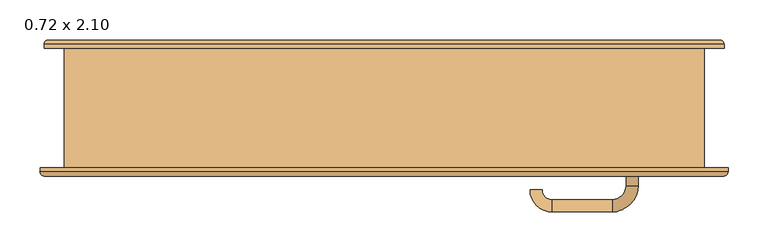
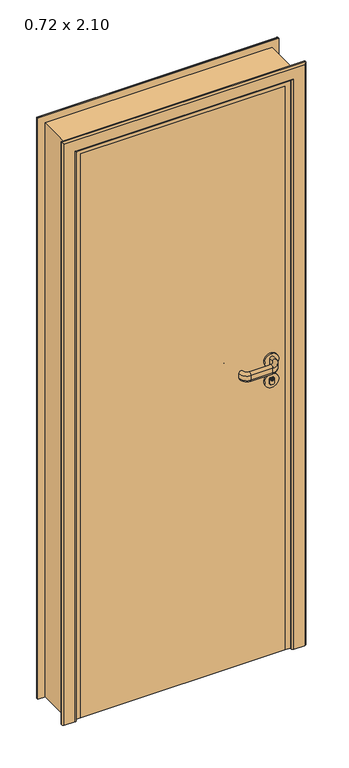
"""IFC4 building model written with IfcOpenShell, lengths in millimetres: door geometry, CC_PORTA ABRIR_1 FOLHA LISA : 0.72 x 2.10."""

import ifcopenshell
import ifcopenshell.guid

model = None  # the IFC model being written
_history = None  # IfcOwnerHistory: only IFC2X3 demands one
_inside = {}  # id of a spatial element -> (the spatial element, [elements in it])
_under = {}  # id of a project, library or spatial element -> (it, [spatial elements below it])
_declared = {}  # id of a project -> (the project, [libraries it declares])
_typed = {}  # id of a type object -> (the type object, [elements of that type])
_made_of = {}  # id of a material, layer set ... -> (it, [elements and type objects made of it])


def new_model(schema):
    """Start an empty IFC model of exactly this schema.

    Asked for "IFC4X3", IfcOpenShell would pick the latest addendum, in which some entities
    have other attributes; the version numbers below select the first issue.
    IFC2X3 requires an IfcOwnerHistory on every rooted entity: one is made here for all.
    """
    global model, _history
    if schema == "IFC4X3":
        model = ifcopenshell.file(schema_version=(4, 3, 0, 0))
    else:
        model = ifcopenshell.file(schema=schema)
    _inside.clear()
    _under.clear()
    _declared.clear()
    _typed.clear()
    _made_of.clear()
    _history = None
    if model.schema == "IFC2X3":
        org = make("IfcOrganization", Name="unknown")
        user = make(
            "IfcPersonAndOrganization",
            ThePerson=make("IfcPerson", FamilyName="unknown"),
            TheOrganization=org,
        )
        app = make(
            "IfcApplication",
            ApplicationDeveloper=org,
            Version="unknown",
            ApplicationFullName="unknown",
            ApplicationIdentifier="unknown",
        )
        _history = make(
            "IfcOwnerHistory",
            OwningUser=user,
            OwningApplication=app,
            ChangeAction="ADDED",
            CreationDate=0,
        )
    return model


def make(cls, **values):
    """One entity of the class cls with the attributes given. An attribute that is None is left unset."""
    return model.create_entity(
        cls, **{name: value for name, value in values.items() if value is not None}
    )


def rooted(cls, **values):
    """An entity with a GlobalId (a new one), such as an element, a storey or a relation."""
    return make(cls, GlobalId=ifcopenshell.guid.new(), OwnerHistory=_history, **values)


def si_unit(unit_type, name, prefix=None):
    """IfcSIUnit, for example si_unit("LENGTHUNIT", "METRE", prefix="MILLI")."""
    return make("IfcSIUnit", UnitType=unit_type, Prefix=prefix, Name=name)


def assignment(units):
    """IfcUnitAssignment: the units of a project."""
    return None if units is None else make("IfcUnitAssignment", Units=units)


def point(xyz):
    """IfcCartesianPoint."""
    return None if xyz is None else make("IfcCartesianPoint", Coordinates=xyz)


def direction(xyz):
    """IfcDirection."""
    return None if xyz is None else make("IfcDirection", DirectionRatios=xyz)


def frame(location, z_axis=None, x_axis=None):
    """IfcAxis2Placement3D, a coordinate frame: its origin and axes. An axis left out is left unset."""
    return make(
        "IfcAxis2Placement3D",
        Location=point(location),
        Axis=direction(z_axis),
        RefDirection=direction(x_axis),
    )


def frame_2d(location, x_axis=None):
    """IfcAxis2Placement2D, a coordinate frame in the plane: its origin and x axis."""
    return make(
        "IfcAxis2Placement2D", Location=point(location), RefDirection=direction(x_axis)
    )


def origin():
    """The frame at (0, 0, 0) with its axes left unset."""
    return frame((0.0, 0.0, 0.0))


def origin_with_axes():
    """The frame at (0, 0, 0) with the z axis (0, 0, 1) and the x axis (1, 0, 0) written out."""
    return frame((0.0, 0.0, 0.0), z_axis=(0.0, 0.0, 1.0), x_axis=(1.0, 0.0, 0.0))


def place(relative_to, where):
    """IfcLocalPlacement: puts the frame where relative to a parent placement (None: the world)."""
    return make(
        "IfcLocalPlacement", PlacementRelTo=relative_to, RelativePlacement=where
    )


def context(
    kind, dimensions, precision=None, world=None, true_north=None, identifier=None
):
    """IfcGeometricRepresentationContext, for example the 3D "Model" context."""
    return make(
        "IfcGeometricRepresentationContext",
        ContextIdentifier=identifier,
        ContextType=kind,
        CoordinateSpaceDimension=dimensions,
        Precision=precision,
        WorldCoordinateSystem=world,
        TrueNorth=true_north,
    )


def project(units=None, contexts=None):
    """IfcProject with its units and contexts."""
    return rooted(
        "IfcProject",
        Name="project",
        RepresentationContexts=contexts,
        UnitsInContext=assignment(units),
    )


def spatial(cls, under=None, at=None, **own):
    """A site, building, storey or space (cls), placed at a placement, below another one or the project."""
    s = rooted(cls, ObjectPlacement=at, **own)
    if under is not None:
        _under.setdefault(under.id(), (under, []))[1].append(s)
    return s


def polyline(points):
    """IfcPolyline through the points."""
    return make("IfcPolyline", Points=[point(p) for p in points])


def circle_curve(where, radius):
    """IfcCircle in the frame where."""
    return make("IfcCircle", Position=where, Radius=radius)


def ellipse_curve(where, semi_axis1, semi_axis2):
    """IfcEllipse in the frame where."""
    return make(
        "IfcEllipse", Position=where, SemiAxis1=semi_axis1, SemiAxis2=semi_axis2
    )


def trimmed(basis, trim1, trim2, sense, master):
    """IfcTrimmedCurve: the piece of a basis curve between two trims."""
    return make(
        "IfcTrimmedCurve",
        BasisCurve=basis,
        Trim1=trim1,
        Trim2=trim2,
        SenseAgreement=sense,
        MasterRepresentation=master,
    )


def segment(curve, same_sense, transition):
    """IfcCompositeCurveSegment."""
    return make(
        "IfcCompositeCurveSegment",
        Transition=transition,
        SameSense=same_sense,
        ParentCurve=curve,
    )


def composite_curve(segments, self_intersect=None):
    """IfcCompositeCurve: segments joined end to end."""
    return make("IfcCompositeCurve", Segments=segments, SelfIntersect=self_intersect)


def outline(outer, holes=None, kind="AREA"):
    """IfcArbitraryClosedProfileDef: a profile drawn as a closed curve; with holes, ...WithVoids."""
    if holes is None:
        return make("IfcArbitraryClosedProfileDef", ProfileType=kind, OuterCurve=outer)
    return make(
        "IfcArbitraryProfileDefWithVoids",
        ProfileType=kind,
        OuterCurve=outer,
        InnerCurves=holes,
    )


def extrude(swept, where, along, depth):
    """IfcExtrudedAreaSolid: the profile swept, set in the frame where, extruded along a direction by depth."""
    return make(
        "IfcExtrudedAreaSolid",
        SweptArea=swept,
        Position=where,
        ExtrudedDirection=direction(along),
        Depth=depth,
    )


def faces_of(points, faces, orient=None, outer=None):
    """IfcFace entities. A face is a list of loops; a loop is a list of indices into points, from 0.

    orient and outer hold one flag for each loop. By default every Orientation is true, the
    first loop of a face is its IfcFaceOuterBound and the others are IfcFaceBound.
    """
    made = []
    for i, loops in enumerate(faces):
        bounds = []
        for j, loop in enumerate(loops):
            is_outer = j == 0 if outer is None else outer[i][j]
            bounds.append(
                make(
                    "IfcFaceOuterBound" if is_outer else "IfcFaceBound",
                    Bound=make("IfcPolyLoop", Polygon=[points[k] for k in loop]),
                    Orientation=True if orient is None else orient[i][j],
                )
            )
        made.append(make("IfcFace", Bounds=bounds))
    return made


def faceted_brep(points, faces, orient=None, outer=None, voids=None):
    """IfcFacetedBrep: a solid bounded by flat faces; with voids (closed shells), ...WithVoids."""
    shared = [point(p) for p in points]
    hull = make("IfcClosedShell", CfsFaces=faces_of(shared, faces, orient, outer))
    if voids is None:
        return make("IfcFacetedBrep", Outer=hull)
    return make(
        "IfcFacetedBrepWithVoids",
        Outer=hull,
        Voids=[
            make(cls, CfsFaces=faces_of(shared, fs, o, b)) for cls, fs, o, b in voids
        ],
    )


def shape(context_of_items, identifier, shape_type, items):
    """IfcShapeRepresentation: the items that make up one representation, for example the "Body"."""
    return make(
        "IfcShapeRepresentation",
        ContextOfItems=context_of_items,
        RepresentationIdentifier=identifier,
        RepresentationType=shape_type,
        Items=items,
    )


def source(mapping_origin, context_of_items, identifier, shape_type, items):
    """IfcRepresentationMap: a shape defined once, which mapped items show again and again."""
    return make(
        "IfcRepresentationMap",
        MappingOrigin=mapping_origin,
        MappedRepresentation=shape(context_of_items, identifier, shape_type, items),
    )


def transform(
    local_origin,
    x_axis=None,
    y_axis=None,
    z_axis=None,
    scale=None,
    scale2=None,
    scale3=None,
    uniform=True,
):
    """IfcCartesianTransformationOperator3D, or its non-uniform kind. x_axis, y_axis, z_axis: its Axis1, 2, 3."""
    if uniform:
        return make(
            "IfcCartesianTransformationOperator3D",
            Axis1=direction(x_axis),
            Axis2=direction(y_axis),
            LocalOrigin=point(local_origin),
            Scale=scale,
            Axis3=direction(z_axis),
        )
    return make(
        "IfcCartesianTransformationOperator3DnonUniform",
        Axis1=direction(x_axis),
        Axis2=direction(y_axis),
        LocalOrigin=point(local_origin),
        Scale=scale,
        Axis3=direction(z_axis),
        Scale2=scale2,
        Scale3=scale3,
    )


def mapped(mapping_source, mapping_target):
    """IfcMappedItem: shows the shape of a source again, moved by a transform."""
    return make(
        "IfcMappedItem", MappingSource=mapping_source, MappingTarget=mapping_target
    )


def made_of(thing, what):
    """Note that an element or type object is made of a material, layer set ...; save() writes the relation."""
    if what is not None:
        _made_of.setdefault(what.id(), (what, []))[1].append(thing)
    return thing


def element(
    cls,
    number,
    at=None,
    inside=None,
    cuts=None,
    type_object=None,
    material=None,
    context=None,
    identifier="Body",
    shape_type=None,
    held_by="IfcProductDefinitionShape",
    body=None,
    shapes=None,
    **own,
):
    """One element of the class cls, such as IfcWall. Its Tag is "e" and its number.

    at: its placement. inside: the storey or other place that contains it. cuts: it is an
    opening in that element (IfcRelVoidsElement). A single representation is given by context,
    identifier, shape_type and body (its items); several are given by shapes. held_by: the class
    of the entity that holds the representations. save() writes the other relations.
    """
    e = rooted(cls, Tag="e%d" % number, ObjectPlacement=at, **own)
    if body is not None:
        shapes = [shape(context, identifier, shape_type, body)]
    if shapes is not None:
        e.Representation = make(held_by, Representations=shapes)
    if inside is not None:
        _inside.setdefault(inside.id(), (inside, []))[1].append(e)
    if cuts is not None:
        rooted(
            "IfcRelVoidsElement", RelatingBuildingElement=cuts, RelatedOpeningElement=e
        )
    if type_object is not None:
        _typed.setdefault(type_object.id(), (type_object, []))[1].append(e)
    return made_of(e, material)


def aggregate(whole, parts):
    """IfcRelAggregates: a whole, such as a stair, and the parts it consists of."""
    return rooted("IfcRelAggregates", RelatingObject=whole, RelatedObjects=parts)


def save(model, path):
    """Write the relations noted so far, then the file.

    IfcRelAggregates (storeys below a building ...), IfcRelContainedInSpatialStructure (elements
    in a storey), IfcRelDefinesByType, IfcRelAssociatesMaterial and IfcRelDeclares: one each for
    every whole, place, type object, material and project.
    """
    for whole, parts in _under.values():
        aggregate(whole, parts)
    for where, things in _inside.values():
        rooted(
            "IfcRelContainedInSpatialStructure",
            RelatedElements=things,
            RelatingStructure=where,
        )
    for kind, things in _typed.values():
        rooted("IfcRelDefinesByType", RelatedObjects=things, RelatingType=kind)
    for what, things in _made_of.values():
        rooted("IfcRelAssociatesMaterial", RelatedObjects=things, RelatingMaterial=what)
    for by, libraries in _declared.values():
        rooted("IfcRelDeclares", RelatingContext=by, RelatedDefinitions=libraries)
    model.write(path)


def plane_surface(at):
    """IfcPlane: the flat surface through the origin of the frame at, square to its z axis."""
    return make("IfcPlane", Position=at)


def cylinder_surface(at, radius):
    """IfcCylindricalSurface: all points at the distance radius from the z axis of the frame at."""
    return make("IfcCylindricalSurface", Position=at, Radius=radius)


def revolved_surface(curve, axis_point, axis_direction):
    """IfcSurfaceOfRevolution: the curve turned about the line through axis_point along axis_direction."""
    return make(
        "IfcSurfaceOfRevolution",
        SweptCurve=make("IfcArbitraryOpenProfileDef", ProfileType="CURVE", Curve=curve),
        AxisPosition=make("IfcAxis1Placement", Location=point(axis_point), Axis=direction(axis_direction)),
    )


def advanced_brep(points, edges, surfaces, faces):
    """IfcAdvancedBrep: a solid bounded by faces that lie on surfaces and meet in shared edges.

    An edge is (start, end): straight between two places in points (the first is 0);
    or (start, end, curve); or (start, end, curve, False) where it runs against its curve.
    A face is (place in surfaces, loops), or (place, loops, False) where it looks against
    its surface's normal. A loop lists edges by number (the first is 1), with a minus sign
    where the edge is run from its end to its start. The first loop is the outer one.
    """
    corners = [point(p) for p in points]
    vertices = [make("IfcVertexPoint", VertexGeometry=c) for c in corners]
    made = []
    for start, end, *more in edges:
        made.append(
            make(
                "IfcEdgeCurve",
                EdgeStart=vertices[start],
                EdgeEnd=vertices[end],
                EdgeGeometry=more[0] if more else make("IfcPolyline", Points=[corners[start], corners[end]]),
                SameSense=more[1] if len(more) > 1 else True,
            )
        )
    hull = []
    for where, loops, *sense in faces:
        bounds = []
        for j, loop in enumerate(loops):
            ring = [make("IfcOrientedEdge", EdgeElement=made[abs(k) - 1], Orientation=k > 0) for k in loop]
            bounds.append(
                make(
                    "IfcFaceOuterBound" if j == 0 else "IfcFaceBound",
                    Bound=make("IfcEdgeLoop", EdgeList=ring),
                    Orientation=True,
                )
            )
        hull.append(make("IfcAdvancedFace", Bounds=bounds, FaceSurface=surfaces[where], SameSense=sense[0] if sense else True))
    return make("IfcAdvancedBrep", Outer=make("IfcClosedShell", CfsFaces=hull))


def door_0_72_x_2_10_8ac540cf(model_context):
    return source(origin(), model_context, "Body", "SolidModel", [
        advanced_brep(
        [(302.5, -40.0, 1091.5062746), (317.5, -40.0, 1091.5062746), (317.5, -40.0, 1108.3826844), (302.5, -40.0, 1108.3826844), (317.5, -18.0, 1091.5062746), (317.5, -18.0, 1108.3826844), (302.5, -18.0, 1108.3826844), (302.5, -18.0, 1091.5062746), (285.0, 14.5, 1108.3826844), (285.0, 14.5, 1091.5062746), (210.0, 14.5, 1091.5062746), (210.0, 14.5, 1108.3826844), (285.0, -0.5, 1091.5062746), (285.0, -0.5, 1108.3826844), (210.0, -0.5, 1108.3826844), (210.0, -0.5, 1091.5062746), (197.5, -13.0, 1091.5062746), (197.5, -13.0, 1108.3826844), (182.5, -13.0, 1108.3826844), (182.5, -13.0, 1091.5062746)],
        [
            (0, 1, circle_curve(frame((310.0, -40.0, 1091.5062746), z_axis=(0.0, -1.0, 0.0), x_axis=(0.0, 0.0, 1.0)), 7.5)),
            (1, 2),
            (2, 3, circle_curve(frame((310.0, -40.0, 1108.3826844), z_axis=(0.0, -1.0, 0.0), x_axis=(0.0, 0.0, 1.0)), 7.5)),
            (3, 0),
            (1, 4),
            (4, 5),
            (5, 2),
            (3, 6),
            (6, 7),
            (7, 0),
            (8, 9),
            (9, 10),
            (10, 11),
            (11, 8),
            (12, 13),
            (13, 14),
            (14, 15),
            (15, 12),
            (7, 4, circle_curve(frame((310.0, -18.0, 1091.5062746), z_axis=(0.0, -1.0, 0.0), x_axis=(0.0, 0.0, 1.0)), 7.5)),
            (5, 6, circle_curve(frame((310.0, -18.0, 1108.3826844), z_axis=(0.0, -1.0, 0.0), x_axis=(0.0, 0.0, 1.0)), 7.5)),
            (9, 12, circle_curve(frame((285.0, 7.0, 1091.5062746), z_axis=(-1.0, 0.0, 0.0), x_axis=(0.0, 0.0, 1.0)), 7.5)),
            (15, 10, circle_curve(frame((210.0, 7.0, 1091.5062746), z_axis=(1.0, 0.0, 0.0), x_axis=(0.0, 0.0, 1.0)), 7.5)),
            (13, 8, circle_curve(frame((285.0, 7.0, 1108.3826844), z_axis=(-1.0, 0.0, 0.0), x_axis=(0.0, 0.0, 1.0)), 7.5)),
            (11, 14, circle_curve(frame((210.0, 7.0, 1108.3826844), z_axis=(1.0, 0.0, 0.0), x_axis=(0.0, 0.0, 1.0)), 7.5)),
            (9, 4, circle_curve(frame((285.0, -18.0, 1091.5062746), z_axis=(0.0, 0.0, -1.0), x_axis=(1.0, 0.0, 0.0)), 32.5)),
            (7, 12, circle_curve(frame((285.0, -18.0, 1091.5062746), z_axis=(0.0, 0.0, 1.0), x_axis=(1.0, 0.0, 0.0)), 17.5)),
            (8, 5, circle_curve(frame((285.0, -18.0, 1108.3826844), z_axis=(0.0, 0.0, -1.0), x_axis=(1.0, 0.0, 0.0)), 32.5)),
            (13, 6, circle_curve(frame((285.0, -18.0, 1108.3826844), z_axis=(0.0, 0.0, -1.0), x_axis=(1.0, 0.0, 0.0)), 17.5)),
            (16, 17),
            (17, 18, circle_curve(frame((190.0, -13.0, 1108.3826844), z_axis=(0.0, -1.0, 0.0), x_axis=(0.0, 0.0, 1.0)), 7.5)),
            (18, 19),
            (19, 16, circle_curve(frame((190.0, -13.0, 1091.5062746), z_axis=(0.0, -1.0, 0.0), x_axis=(0.0, 0.0, 1.0)), 7.5)),
            (19, 10, circle_curve(frame((210.0, -13.0, 1091.5062746), z_axis=(0.0, 0.0, -1.0), x_axis=(0.0, 1.0, 0.0)), 27.5)),
            (15, 16, circle_curve(frame((210.0, -13.0, 1091.5062746), z_axis=(0.0, 0.0, 1.0), x_axis=(0.0, 1.0, 0.0)), 12.5)),
            (18, 11, circle_curve(frame((210.0, -13.0, 1108.3826844), z_axis=(0.0, 0.0, -1.0), x_axis=(0.0, 1.0, 0.0)), 27.5)),
            (17, 14, circle_curve(frame((210.0, -13.0, 1108.3826844), z_axis=(0.0, 0.0, -1.0), x_axis=(0.0, 1.0, 0.0)), 12.5)),
        ],
        [
            plane_surface(frame((310.0, -40.0, 1099.9444795), z_axis=(0.0, -1.0, 0.0), x_axis=(0.0, 0.0, 1.0))),
            plane_surface(frame((317.5, -40.0, 1091.5062746), z_axis=(1.0, 0.0, 0.0), x_axis=(0.0, 1.0, 0.0))),
            plane_surface(frame((302.5, -40.0, 1108.3826844), z_axis=(-1.0, 0.0, 0.0), x_axis=(0.0, 1.0, 0.0))),
            plane_surface(frame((285.0, 14.5, 1091.5062746), z_axis=(0.0, 1.0, 0.0), x_axis=(-1.0, 0.0, 0.0))),
            plane_surface(frame((285.0, -0.5, 1108.3826844), z_axis=(0.0, -1.0, 0.0), x_axis=(-1.0, 0.0, 0.0))),
            cylinder_surface(frame((310.0, -40.0, 1091.5062746), z_axis=(0.0, -1.0, 0.0), x_axis=(0.0, 0.0, 1.0)), 7.5),
            cylinder_surface(frame((310.0, -40.0, 1108.3826844), z_axis=(0.0, -1.0, 0.0), x_axis=(0.0, 0.0, 1.0)), 7.5),
            cylinder_surface(frame((285.0, 7.0, 1091.5062746), z_axis=(1.0, 0.0, 0.0), x_axis=(0.0, 0.0, 1.0)), 7.5),
            cylinder_surface(frame((285.0, 7.0, 1108.3826844), z_axis=(1.0, 0.0, 0.0), x_axis=(0.0, 0.0, 1.0)), 7.5),
            revolved_surface(trimmed(ellipse_curve(frame((310.0, -18.0, 1091.5062746), z_axis=(0.0, -1.0, 0.0), x_axis=(0.0, 0.0, 1.0)), 7.5, 7.5), [point((302.5, -18.0, 1091.5062746))], [point((317.5, -18.0, 1091.5062746))], True, "CARTESIAN"), (285.0, -18.0, 1099.9444795), (0.0, 0.0, 1.0)),
            cylinder_surface(frame((285.0, -18.0, 1099.9444795), z_axis=(0.0, 0.0, 1.0), x_axis=(1.0, 0.0, 0.0)), 32.5),
            revolved_surface(trimmed(ellipse_curve(frame((310.0, -18.0, 1108.3826844), z_axis=(0.0, -1.0, 0.0), x_axis=(0.0, 0.0, 1.0)), 7.5, 7.5), [point((317.5, -18.0, 1108.3826844))], [point((302.5, -18.0, 1108.3826844))], True, "CARTESIAN"), (285.0, -18.0, 1099.9444795), (0.0, 0.0, 1.0)),
            revolved_surface(polyline([(302.5, -18.0, 1108.3826844), (302.5, -18.0, 1091.5062746)]), (285.0, -18.0, 1099.9444795), (0.0, 0.0, 1.0)),
            plane_surface(frame((190.0, -13.0, 1099.9444795), z_axis=(0.0, -1.0, 0.0), x_axis=(0.0, 0.0, 1.0))),
            revolved_surface(trimmed(ellipse_curve(frame((210.0, 7.0, 1091.5062746), z_axis=(1.0, 0.0, 0.0), x_axis=(0.0, 0.0, 1.0)), 7.5, 7.5), [point((210.0, -0.5, 1091.5062746))], [point((210.0, 14.5, 1091.5062746))], True, "CARTESIAN"), (210.0, -13.0, 1099.9444795), (0.0, 0.0, 1.0)),
            cylinder_surface(frame((210.0, -13.0, 1099.9444795), z_axis=(0.0, 0.0, 1.0), x_axis=(0.0, 1.0, 0.0)), 27.5),
            revolved_surface(trimmed(ellipse_curve(frame((210.0, 7.0, 1108.3826844), z_axis=(1.0, 0.0, 0.0), x_axis=(0.0, 0.0, 1.0)), 7.5, 7.5), [point((210.0, 14.5, 1108.3826844))], [point((210.0, -0.5, 1108.3826844))], True, "CARTESIAN"), (210.0, -13.0, 1099.9444795), (0.0, 0.0, 1.0)),
            revolved_surface(polyline([(210.0, -0.5, 1108.3826844), (210.0, -0.5, 1091.5062746)]), (210.0, -13.0, 1099.9444795), (0.0, 0.0, 1.0)),
        ],
        [
            (0, [[1, 2, 3, 4]]),
            (1, [[-2, 5, 6, 7]]),
            (2, [[-4, 8, 9, 10]]),
            (3, [[11, 12, 13, 14]]),
            (4, [[15, 16, 17, 18]]),
            (5, [[-1, -10, 19, -5]]),
            (6, [[-3, -7, 20, -8]]),
            (7, [[21, -18, 22, -12]]),
            (8, [[23, -14, 24, -16]]),
            (9, [[25, -19, 26, -21]]),
            (10, [[27, -6, -25, -11]]),
            (11, [[28, -20, -27, -23]]),
            (12, [[-26, -9, -28, -15]]),
            (13, [[29, 30, 31, 32]]),
            (14, [[33, -22, 34, -32]]),
            (15, [[35, -13, -33, -31]]),
            (16, [[36, -24, -35, -30]]),
            (17, [[-34, -17, -36, -29]]),
        ],
    ),
        extrude(outline(polyline([(311.0, -40.0), (309.0, -40.0), (309.0, -30.9), (311.0, -30.9), (311.0, -40.0)])), frame((0.0, 0.0, 1027.9555433), z_axis=(0.0, 0.0, 1.0), x_axis=(1.0, 0.0, 0.0)), (0.0, 0.0, 1.0), 7.8071257),
        extrude(outline(composite_curve([segment(trimmed(circle_curve(frame_2d((1031.5611613, 310.0)), 5.0), [point((1036.5611613, 310.0))], [point((1026.5611613, 310.0))], False, "CARTESIAN"), True, "CONTINUOUS"), segment(trimmed(circle_curve(frame_2d((1031.5611613, 310.0)), 5.0), [point((1026.5611613, 310.0))], [point((1036.5611613, 310.0))], False, "CARTESIAN"), True, "CONTINUOUS")], self_intersect=False), holes=[polyline([(1035.7626689, 311.0), (1027.9555433, 311.0), (1027.9555433, 309.0), (1035.7626689, 309.0), (1035.7626689, 311.0)])]), frame((0.0, -40.0, 0.0), z_axis=(0.0, 1.0, 0.0), x_axis=(0.0, 0.0, 1.0)), (0.0, 0.0, 1.0), 10.0),
        extrude(outline(composite_curve([segment(polyline([(1033.4817325, 302.5), (1016.4817325, 302.5)]), True, "CONTINUOUS"), segment(trimmed(circle_curve(frame_2d((1016.4817325, 306.5)), 4.0), [point((1016.4817325, 302.5))], [point((1012.4817325, 306.5))], False, "CARTESIAN"), True, "CONTINUOUS"), segment(polyline([(1012.4817325, 306.5), (1012.4817325, 313.5)]), True, "CONTINUOUS"), segment(trimmed(circle_curve(frame_2d((1016.4817325, 313.5)), 4.0), [point((1012.4817325, 313.5))], [point((1016.4817325, 317.5))], False, "CARTESIAN"), True, "CONTINUOUS"), segment(polyline([(1016.4817325, 317.5), (1033.4817325, 317.5)]), True, "CONTINUOUS"), segment(trimmed(circle_curve(frame_2d((1033.4817325, 313.5)), 4.0), [point((1033.4817325, 317.5))], [point((1037.4817325, 313.5))], False, "CARTESIAN"), True, "CONTINUOUS"), segment(polyline([(1037.4817325, 313.5), (1037.4817325, 306.5)]), True, "CONTINUOUS"), segment(trimmed(circle_curve(frame_2d((1033.4817325, 306.5)), 4.0), [point((1037.4817325, 306.5))], [point((1033.4817325, 302.5))], False, "CARTESIAN"), True, "CONTINUOUS")], self_intersect=False)), frame((0.0, -40.0, 0.0), z_axis=(0.0, 1.0, 0.0), x_axis=(0.0, 0.0, 1.0)), (0.0, 0.0, 1.0), 9.0),
        extrude(outline(composite_curve([segment(trimmed(circle_curve(frame_2d((1099.9444795, 310.0)), 25.0), [point((1124.9444795, 310.0))], [point((1074.9444795, 310.0))], False, "CARTESIAN"), True, "CONTINUOUS"), segment(trimmed(circle_curve(frame_2d((1099.9444795, 310.0)), 25.0), [point((1074.9444795, 310.0))], [point((1124.9444795, 310.0))], False, "CARTESIAN"), True, "CONTINUOUS")], self_intersect=False)), frame((0.0, -40.0, 0.0), z_axis=(0.0, 1.0, 0.0), x_axis=(0.0, 0.0, 1.0)), (0.0, 0.0, 1.0), 6.0),
        extrude(outline(composite_curve([segment(trimmed(circle_curve(frame_2d((1024.9444795, 310.0)), 25.0), [point((1049.9444795, 310.0))], [point((999.9444795, 310.0))], False, "CARTESIAN"), True, "CONTINUOUS"), segment(trimmed(circle_curve(frame_2d((1024.9444795, 310.0)), 25.0), [point((999.9444795, 310.0))], [point((1049.9444795, 310.0))], False, "CARTESIAN"), True, "CONTINUOUS")], self_intersect=False), holes=[composite_curve([segment(trimmed(circle_curve(frame_2d((1033.4817325, 313.5)), 4.0), [point((1037.4817325, 313.5))], [point((1033.4817325, 317.5))], True, "CARTESIAN"), True, "CONTINUOUS"), segment(polyline([(1033.4817325, 317.5), (1016.4817325, 317.5)]), True, "CONTINUOUS"), segment(trimmed(circle_curve(frame_2d((1016.4817325, 313.5)), 4.0), [point((1016.4817325, 317.5))], [point((1012.4817325, 313.5))], True, "CARTESIAN"), True, "CONTINUOUS"), segment(polyline([(1012.4817325, 313.5), (1012.4817325, 306.5)]), True, "CONTINUOUS"), segment(trimmed(circle_curve(frame_2d((1016.4817325, 306.5)), 4.0), [point((1012.4817325, 306.5))], [point((1016.4817325, 302.5))], True, "CARTESIAN"), True, "CONTINUOUS"), segment(polyline([(1016.4817325, 302.5), (1033.4817325, 302.5)]), True, "CONTINUOUS"), segment(trimmed(circle_curve(frame_2d((1033.4817325, 306.5)), 4.0), [point((1033.4817325, 302.5))], [point((1037.4817325, 306.5))], True, "CARTESIAN"), True, "CONTINUOUS"), segment(polyline([(1037.4817325, 306.5), (1037.4817325, 313.5)]), True, "CONTINUOUS")], self_intersect=False)]), frame((0.0, -40.0, 0.0), z_axis=(0.0, 1.0, 0.0), x_axis=(0.0, 0.0, 1.0)), (0.0, 0.0, 1.0), 6.0),
        extrude(outline(polyline([(311.0, -84.1), (309.0, -84.1), (309.0, -75.0), (311.0, -75.0), (311.0, -84.1)])), frame((0.0, 0.0, 1027.9555433), z_axis=(0.0, 0.0, 1.0), x_axis=(1.0, 0.0, 0.0)), (0.0, 0.0, 1.0), 7.8071257),
        advanced_brep(
        [(310.0, -85.0, 1036.5611613), (310.0, -85.0, 1026.5611613), (311.0, -85.0, 1035.7626689), (311.0, -85.0, 1027.9555433), (309.0, -85.0, 1027.9555433), (309.0, -85.0, 1035.7626689), (310.0, -75.0, 1049.9444795), (310.0, -75.0, 999.9444795), (310.0, -84.0, 1036.5611613), (310.0, -84.0, 1026.5611613), (311.0, -84.0, 1035.7626689), (311.0, -84.0, 1027.9555433), (309.0, -84.0, 1027.9555433), (309.0, -84.0, 1035.7626689), (302.5, -84.0, 1033.4817325), (302.5, -84.0, 1016.4817325), (306.5, -84.0, 1012.4817325), (313.5, -84.0, 1012.4817325), (317.5, -84.0, 1016.4817325), (317.5, -84.0, 1033.4817325), (313.5, -84.0, 1037.4817325), (306.5, -84.0, 1037.4817325), (302.5, -81.0, 1033.4817325), (302.5, -81.0, 1016.4817325), (306.5, -81.0, 1012.4817325), (313.5, -81.0, 1012.4817325), (317.5, -81.0, 1016.4817325), (317.5, -81.0, 1033.4817325), (313.5, -81.0, 1037.4817325), (306.5, -81.0, 1037.4817325), (310.0, -81.0, 1049.9444795), (310.0, -81.0, 999.9444795)],
        [
            (0, 1, circle_curve(frame((310.0, -85.0, 1031.5611613), z_axis=(0.0, -1.0, 0.0), x_axis=(0.0, 0.0, -1.0)), 5.0)),
            (1, 0, circle_curve(frame((310.0, -85.0, 1031.5611613), z_axis=(0.0, -1.0, 0.0), x_axis=(0.0, 0.0, -1.0)), 5.0)),
            (2, 3),
            (3, 4),
            (4, 5),
            (5, 2),
            (6, 7, circle_curve(frame((310.0, -75.0, 1024.9444795), z_axis=(0.0, 1.0, 0.0), x_axis=(0.0, 0.0, -1.0)), 25.0)),
            (7, 6, circle_curve(frame((310.0, -75.0, 1024.9444795), z_axis=(0.0, 1.0, 0.0), x_axis=(0.0, 0.0, -1.0)), 25.0)),
            (0, 8),
            (8, 9, circle_curve(frame((310.0, -84.0, 1031.5611613), z_axis=(0.0, -1.0, 0.0), x_axis=(0.0, 0.0, -1.0)), 5.0)),
            (9, 1),
            (9, 8, circle_curve(frame((310.0, -84.0, 1031.5611613), z_axis=(0.0, -1.0, 0.0), x_axis=(0.0, 0.0, -1.0)), 5.0)),
            (2, 10),
            (10, 11),
            (11, 3),
            (11, 12),
            (12, 4),
            (12, 13),
            (13, 5),
            (13, 10),
            (14, 15),
            (15, 16, circle_curve(frame((306.5, -84.0, 1016.4817325), z_axis=(0.0, -1.0, 0.0), x_axis=(0.0, 0.0, -1.0)), 4.0)),
            (16, 17),
            (17, 18, circle_curve(frame((313.5, -84.0, 1016.4817325), z_axis=(0.0, -1.0, 0.0), x_axis=(0.0, 0.0, -1.0)), 4.0)),
            (18, 19),
            (19, 20, circle_curve(frame((313.5, -84.0, 1033.4817325), z_axis=(0.0, -1.0, 0.0), x_axis=(0.0, 0.0, -1.0)), 4.0)),
            (20, 21),
            (21, 14, circle_curve(frame((306.5, -84.0, 1033.4817325), z_axis=(0.0, -1.0, 0.0), x_axis=(0.0, 0.0, -1.0)), 4.0)),
            (14, 22),
            (22, 23),
            (23, 15),
            (23, 24, circle_curve(frame((306.5, -81.0, 1016.4817325), z_axis=(0.0, -1.0, 0.0), x_axis=(0.0, 0.0, -1.0)), 4.0)),
            (24, 16),
            (24, 25),
            (25, 17),
            (25, 26, circle_curve(frame((313.5, -81.0, 1016.4817325), z_axis=(0.0, -1.0, 0.0), x_axis=(0.0, 0.0, -1.0)), 4.0)),
            (26, 18),
            (26, 27),
            (27, 19),
            (27, 28, circle_curve(frame((313.5, -81.0, 1033.4817325), z_axis=(0.0, -1.0, 0.0), x_axis=(0.0, 0.0, -1.0)), 4.0)),
            (28, 20),
            (28, 29),
            (29, 21),
            (29, 22, circle_curve(frame((306.5, -81.0, 1033.4817325), z_axis=(0.0, -1.0, 0.0), x_axis=(0.0, 0.0, -1.0)), 4.0)),
            (30, 31, circle_curve(frame((310.0, -81.0, 1024.9444795), z_axis=(0.0, -1.0, 0.0), x_axis=(0.0, 0.0, -1.0)), 25.0)),
            (31, 30, circle_curve(frame((310.0, -81.0, 1024.9444795), z_axis=(0.0, -1.0, 0.0), x_axis=(0.0, 0.0, -1.0)), 25.0)),
            (30, 6),
            (7, 31),
        ],
        [
            plane_surface(frame((310.0, -85.0, 1026.5611613), z_axis=(0.0, -1.0, 0.0), x_axis=(1.0, 0.0, 0.0))),
            plane_surface(frame((310.0, -75.0, 1026.5611613), z_axis=(0.0, 1.0, 0.0), x_axis=(-1.0, 0.0, 0.0))),
            cylinder_surface(frame((310.0, -75.0, 1031.5611613), z_axis=(0.0, -1.0, 0.0), x_axis=(0.0, 0.0, -1.0)), 5.0),
            plane_surface(frame((311.0, -85.0, 1035.7626689), z_axis=(-1.0, 0.0, 0.0), x_axis=(0.0, 1.0, 0.0))),
            plane_surface(frame((311.0, -85.0, 1027.9555433), z_axis=(0.0, 0.0, 1.0), x_axis=(0.0, 1.0, 0.0))),
            plane_surface(frame((309.0, -85.0, 1027.9555433), z_axis=(1.0, 0.0, 0.0), x_axis=(0.0, 1.0, 0.0))),
            plane_surface(frame((309.0, -85.0, 1035.7626689), z_axis=(0.0, 0.0, -1.0), x_axis=(0.0, 1.0, 0.0))),
            plane_surface(frame((302.5, -84.0, 1016.4817325), z_axis=(0.0, -1.0, 0.0), x_axis=(0.0, 0.0, -1.0))),
            plane_surface(frame((302.5, -84.0, 1033.4817325), z_axis=(-1.0, 0.0, 0.0), x_axis=(0.0, 1.0, 0.0))),
            cylinder_surface(frame((306.5, -75.0, 1016.4817325), z_axis=(0.0, -1.0, 0.0), x_axis=(0.0, 0.0, -1.0)), 4.0),
            plane_surface(frame((306.5, -84.0, 1012.4817325), z_axis=(0.0, 0.0, -1.0), x_axis=(0.0, 1.0, 0.0))),
            cylinder_surface(frame((313.5, -75.0, 1016.4817325), z_axis=(0.0, -1.0, 0.0), x_axis=(0.0, 0.0, -1.0)), 4.0),
            plane_surface(frame((317.5, -84.0, 1016.4817325), z_axis=(1.0, 0.0, 0.0), x_axis=(0.0, 1.0, 0.0))),
            cylinder_surface(frame((313.5, -75.0, 1033.4817325), z_axis=(0.0, -1.0, 0.0), x_axis=(0.0, 0.0, -1.0)), 4.0),
            plane_surface(frame((313.5, -84.0, 1037.4817325), z_axis=(0.0, 0.0, 1.0), x_axis=(0.0, 1.0, 0.0))),
            cylinder_surface(frame((306.5, -75.0, 1033.4817325), z_axis=(0.0, -1.0, 0.0), x_axis=(0.0, 0.0, -1.0)), 4.0),
            plane_surface(frame((310.0, -81.0, 1074.9444795), z_axis=(0.0, -1.0, 0.0), x_axis=(1.0, 0.0, 0.0))),
            cylinder_surface(frame((310.0, -75.0, 1024.9444795), z_axis=(0.0, -1.0, 0.0), x_axis=(0.0, 0.0, -1.0)), 25.0),
        ],
        [
            (0, [[1, 2], [3, 4, 5, 6]]),
            (1, [[7, 8]]),
            (2, [[-1, 9, 10, 11]]),
            (2, [[-2, -11, 12, -9]]),
            (3, [[-3, 13, 14, 15]]),
            (4, [[-4, -15, 16, 17]]),
            (5, [[-5, -17, 18, 19]]),
            (6, [[-6, -19, 20, -13]]),
            (7, [[-14, -20, -18, -16]]),
            (7, [[21, 22, 23, 24, 25, 26, 27, 28], [-10, -12]]),
            (8, [[-21, 29, 30, 31]]),
            (9, [[-22, -31, 32, 33]]),
            (10, [[-23, -33, 34, 35]]),
            (11, [[-24, -35, 36, 37]]),
            (12, [[-25, -37, 38, 39]]),
            (13, [[-26, -39, 40, 41]]),
            (14, [[-27, -41, 42, 43]]),
            (15, [[-28, -43, 44, -29]]),
            (16, [[45, 46], [-30, -44, -42, -40, -38, -36, -34, -32]]),
            (17, [[-45, 47, -8, 48]]),
            (17, [[-46, -48, -7, -47]]),
        ],
    ),
        advanced_brep(
        [(310.0, -75.0, 1124.9444795), (310.0, -75.0, 1074.9444795), (310.0, -81.0, 1124.9444795), (310.0, -81.0, 1074.9444795)],
        [
            (0, 1, circle_curve(frame((310.0, -75.0, 1099.9444795), z_axis=(0.0, 1.0, 0.0), x_axis=(0.0, 0.0, -1.0)), 25.0)),
            (1, 0, circle_curve(frame((310.0, -75.0, 1099.9444795), z_axis=(0.0, 1.0, 0.0), x_axis=(0.0, 0.0, -1.0)), 25.0)),
            (2, 3, circle_curve(frame((310.0, -81.0, 1099.9444795), z_axis=(0.0, -1.0, 0.0), x_axis=(0.0, 0.0, -1.0)), 25.0)),
            (3, 2, circle_curve(frame((310.0, -81.0, 1099.9444795), z_axis=(0.0, -1.0, 0.0), x_axis=(0.0, 0.0, -1.0)), 25.0)),
            (2, 0),
            (1, 3),
        ],
        [
            plane_surface(frame((310.0, -75.0, 1026.5611613), z_axis=(0.0, 1.0, 0.0), x_axis=(-1.0, 0.0, 0.0))),
            plane_surface(frame((310.0, -81.0, 1074.9444795), z_axis=(0.0, -1.0, 0.0), x_axis=(1.0, 0.0, 0.0))),
            cylinder_surface(frame((310.0, -75.0, 1099.9444795), z_axis=(0.0, -1.0, 0.0), x_axis=(0.0, 0.0, -1.0)), 25.0),
        ],
        [
            (0, [[1, 2]]),
            (1, [[3, 4]]),
            (2, [[-3, 5, -2, 6]]),
            (2, [[-4, -6, -1, -5]]),
        ],
    ),
        advanced_brep(
        [(302.5, -75.0, 1108.4382049), (317.5, -75.0, 1108.4382049), (317.5, -75.0, 1091.5617951), (302.5, -75.0, 1091.5617951), (317.5, -97.0, 1108.4382049), (317.5, -97.0, 1091.5617951), (302.5, -97.0, 1091.5617951), (302.5, -97.0, 1108.4382049), (285.0, -129.5, 1091.5617951), (285.0, -129.5, 1108.4382049), (210.0, -129.5, 1108.4382049), (210.0, -129.5, 1091.5617951), (285.0, -114.5, 1108.4382049), (285.0, -114.5, 1091.5617951), (210.0, -114.5, 1091.5617951), (210.0, -114.5, 1108.4382049), (197.5, -102.0, 1108.4382049), (197.5, -102.0, 1091.5617951), (182.5, -102.0, 1091.5617951), (182.5, -102.0, 1108.4382049)],
        [
            (0, 1, circle_curve(frame((310.0, -75.0, 1108.4382049), z_axis=(0.0, 1.0, 0.0), x_axis=(-1.0, 0.0, 0.0)), 7.5)),
            (1, 2),
            (2, 3, circle_curve(frame((310.0, -75.0, 1091.5617951), z_axis=(0.0, 1.0, 0.0), x_axis=(-1.0, 0.0, 0.0)), 7.5)),
            (3, 0),
            (1, 4),
            (4, 5),
            (5, 2),
            (3, 6),
            (6, 7),
            (7, 0),
            (8, 9),
            (9, 10),
            (10, 11),
            (11, 8),
            (12, 13),
            (13, 14),
            (14, 15),
            (15, 12),
            (7, 4, circle_curve(frame((310.0, -97.0, 1108.4382049), z_axis=(0.0, 1.0, 0.0), x_axis=(-1.0, 0.0, 0.0)), 7.5)),
            (5, 6, circle_curve(frame((310.0, -97.0, 1091.5617951), z_axis=(0.0, 1.0, 0.0), x_axis=(-1.0, 0.0, 0.0)), 7.5)),
            (9, 12, circle_curve(frame((285.0, -122.0, 1108.4382049), z_axis=(-1.0, 0.0, 0.0), x_axis=(0.0, 1.0, 0.0)), 7.5)),
            (15, 10, circle_curve(frame((210.0, -122.0, 1108.4382049), z_axis=(1.0, 0.0, 0.0), x_axis=(0.0, 1.0, 0.0)), 7.5)),
            (13, 8, circle_curve(frame((285.0, -122.0, 1091.5617951), z_axis=(-1.0, 0.0, 0.0), x_axis=(0.0, 1.0, 0.0)), 7.5)),
            (11, 14, circle_curve(frame((210.0, -122.0, 1091.5617951), z_axis=(1.0, 0.0, 0.0), x_axis=(0.0, 1.0, 0.0)), 7.5)),
            (9, 4, circle_curve(frame((285.0, -97.0, 1108.4382049), z_axis=(0.0, 0.0, 1.0), x_axis=(1.0, 0.0, 0.0)), 32.5)),
            (7, 12, circle_curve(frame((285.0, -97.0, 1108.4382049), z_axis=(0.0, 0.0, -1.0), x_axis=(1.0, 0.0, 0.0)), 17.5)),
            (8, 5, circle_curve(frame((285.0, -97.0, 1091.5617951), z_axis=(0.0, 0.0, 1.0), x_axis=(1.0, 0.0, 0.0)), 32.5)),
            (13, 6, circle_curve(frame((285.0, -97.0, 1091.5617951), z_axis=(0.0, 0.0, 1.0), x_axis=(1.0, 0.0, 0.0)), 17.5)),
            (16, 17),
            (17, 18, circle_curve(frame((190.0, -102.0, 1091.5617951), z_axis=(0.0, 1.0, 0.0), x_axis=(1.0, 0.0, 0.0)), 7.5)),
            (18, 19),
            (19, 16, circle_curve(frame((190.0, -102.0, 1108.4382049), z_axis=(0.0, 1.0, 0.0), x_axis=(1.0, 0.0, 0.0)), 7.5)),
            (19, 10, circle_curve(frame((210.0, -102.0, 1108.4382049), z_axis=(0.0, 0.0, 1.0), x_axis=(0.0, -1.0, 0.0)), 27.5)),
            (15, 16, circle_curve(frame((210.0, -102.0, 1108.4382049), z_axis=(0.0, 0.0, -1.0), x_axis=(0.0, -1.0, 0.0)), 12.5)),
            (18, 11, circle_curve(frame((210.0, -102.0, 1091.5617951), z_axis=(0.0, 0.0, 1.0), x_axis=(0.0, -1.0, 0.0)), 27.5)),
            (17, 14, circle_curve(frame((210.0, -102.0, 1091.5617951), z_axis=(0.0, 0.0, 1.0), x_axis=(0.0, -1.0, 0.0)), 12.5)),
        ],
        [
            plane_surface(frame((310.0, -75.0, 1100.0), z_axis=(0.0, 1.0, 0.0), x_axis=(0.0, 0.0, -1.0))),
            plane_surface(frame((317.5, -75.0, 1108.4382049), z_axis=(1.0, 0.0, 0.0), x_axis=(0.0, -1.0, 0.0))),
            plane_surface(frame((302.5, -75.0, 1091.5617951), z_axis=(-1.0, 0.0, 0.0), x_axis=(0.0, -1.0, 0.0))),
            plane_surface(frame((285.0, -129.5, 1108.4382049), z_axis=(0.0, -1.0, 0.0), x_axis=(-1.0, 0.0, 0.0))),
            plane_surface(frame((285.0, -114.5, 1091.5617951), z_axis=(0.0, 1.0, 0.0), x_axis=(-1.0, 0.0, 0.0))),
            cylinder_surface(frame((310.0, -75.0, 1108.4382049), z_axis=(0.0, 1.0, 0.0), x_axis=(-1.0, 0.0, 0.0)), 7.5),
            cylinder_surface(frame((310.0, -75.0, 1091.5617951), z_axis=(0.0, 1.0, 0.0), x_axis=(-1.0, 0.0, 0.0)), 7.5),
            cylinder_surface(frame((285.0, -122.0, 1108.4382049), z_axis=(1.0, 0.0, 0.0), x_axis=(0.0, 1.0, 0.0)), 7.5),
            cylinder_surface(frame((285.0, -122.0, 1091.5617951), z_axis=(1.0, 0.0, 0.0), x_axis=(0.0, 1.0, 0.0)), 7.5),
            revolved_surface(trimmed(ellipse_curve(frame((310.0, -97.0, 1108.4382049), z_axis=(0.0, 1.0, 0.0), x_axis=(-1.0, 0.0, 0.0)), 7.5, 7.5), [point((302.5, -97.0, 1108.4382049))], [point((317.5, -97.0, 1108.4382049))], True, "CARTESIAN"), (285.0, -97.0, 1100.0), (0.0, 0.0, -1.0)),
            cylinder_surface(frame((285.0, -97.0, 1100.0), z_axis=(0.0, 0.0, -1.0), x_axis=(1.0, 0.0, 0.0)), 32.5),
            revolved_surface(trimmed(ellipse_curve(frame((310.0, -97.0, 1091.5617951), z_axis=(0.0, 1.0, 0.0), x_axis=(-1.0, 0.0, 0.0)), 7.5, 7.5), [point((317.5, -97.0, 1091.5617951))], [point((302.5, -97.0, 1091.5617951))], True, "CARTESIAN"), (285.0, -97.0, 1100.0), (0.0, 0.0, -1.0)),
            revolved_surface(polyline([(302.5, -97.0, 1091.5617951), (302.5, -97.0, 1108.4382049)]), (285.0, -97.0, 1100.0), (0.0, 0.0, -1.0)),
            plane_surface(frame((190.0, -102.0, 1100.0), z_axis=(0.0, 1.0, 0.0), x_axis=(0.0, 0.0, -1.0))),
            revolved_surface(trimmed(ellipse_curve(frame((210.0, -122.0, 1108.4382049), z_axis=(1.0, 0.0, 0.0), x_axis=(0.0, 1.0, 0.0)), 7.5, 7.5), [point((210.0, -114.5, 1108.4382049))], [point((210.0, -129.5, 1108.4382049))], True, "CARTESIAN"), (210.0, -102.0, 1100.0), (0.0, 0.0, -1.0)),
            cylinder_surface(frame((210.0, -102.0, 1100.0), z_axis=(0.0, 0.0, -1.0), x_axis=(0.0, -1.0, 0.0)), 27.5),
            revolved_surface(trimmed(ellipse_curve(frame((210.0, -122.0, 1091.5617951), z_axis=(1.0, 0.0, 0.0), x_axis=(0.0, 1.0, 0.0)), 7.5, 7.5), [point((210.0, -129.5, 1091.5617951))], [point((210.0, -114.5, 1091.5617951))], True, "CARTESIAN"), (210.0, -102.0, 1100.0), (0.0, 0.0, -1.0)),
            revolved_surface(polyline([(210.0, -114.5, 1091.5617951), (210.0, -114.5, 1108.4382049)]), (210.0, -102.0, 1100.0), (0.0, 0.0, -1.0)),
        ],
        [
            (0, [[1, 2, 3, 4]]),
            (1, [[-2, 5, 6, 7]]),
            (2, [[-4, 8, 9, 10]]),
            (3, [[11, 12, 13, 14]]),
            (4, [[15, 16, 17, 18]]),
            (5, [[-1, -10, 19, -5]]),
            (6, [[-3, -7, 20, -8]]),
            (7, [[21, -18, 22, -12]]),
            (8, [[23, -14, 24, -16]]),
            (9, [[25, -19, 26, -21]]),
            (10, [[27, -6, -25, -11]]),
            (11, [[28, -20, -27, -23]]),
            (12, [[-26, -9, -28, -15]]),
            (13, [[29, 30, 31, 32]]),
            (14, [[33, -22, 34, -32]]),
            (15, [[35, -13, -33, -31]]),
            (16, [[36, -24, -35, -30]]),
            (17, [[-34, -17, -36, -29]]),
        ],
    ),
        extrude(outline(polyline([(360.0, -75.0), (-360.0, -75.0), (-360.0, -40.0), (360.0, -40.0), (360.0, -75.0)])), origin_with_axes(), (0.0, 0.0, 1.0), 2100.0),
        advanced_brep(
        [(-380.5, 85.0, 0.0), (-375.0, 79.5, 0.0), (-375.0, 75.0, 0.0), (-425.0, 75.0, 0.0), (-425.0, 79.500573, 0.0), (-419.500573, 85.0, 0.0), (-380.5, 85.0, 2120.5), (-375.0, 79.5, 2115.0), (-375.0, 75.0, 2115.0), (375.0, 75.0, 2115.0), (375.0, 75.0, 0.0), (425.0, 75.0, 0.0), (425.0, 75.0, 2165.0), (-425.0, 75.0, 2165.0), (-425.0, 79.500573, 2165.0), (-419.500573, 85.0, 2159.500573), (419.500573, 85.0, 2159.500573), (419.500573, 85.0, 0.0), (380.5, 85.0, 0.0), (380.5, 85.0, 2120.5), (375.0, 79.5, 2115.0), (375.0, 79.5, 0.0), (425.0, 79.500573, 0.0), (425.0, 79.500573, 2165.0)],
        [
            (0, 1, circle_curve(frame((-380.5, 79.5, 0.0), z_axis=(0.0, 0.0, -1.0), x_axis=(0.0, 1.0, 0.0)), 5.5)),
            (1, 2),
            (2, 3),
            (3, 4),
            (4, 5, circle_curve(frame((-419.500573, 79.500573, 0.0), z_axis=(0.0, 0.0, -1.0), x_axis=(0.0, 1.0, 0.0)), 5.499427)),
            (5, 0),
            (0, 6),
            (6, 7, ellipse_curve(frame((-380.5, 79.5, 2120.5), z_axis=(-0.7071067811865475, 0.0, -0.7071067811865476), x_axis=(0.7071067811865476, 0.0, -0.7071067811865474)), 7.7781746, 5.5)),
            (7, 1),
            (7, 8),
            (8, 2),
            (8, 9),
            (9, 10),
            (10, 11),
            (11, 12),
            (12, 13),
            (13, 3),
            (13, 14),
            (14, 4),
            (14, 15, ellipse_curve(frame((-419.500573, 79.500573, 2159.500573), z_axis=(-0.7071067811865475, 0.0, -0.7071067811865476), x_axis=(0.7071067811865476, 0.0, -0.7071067811865474)), 7.7773642, 5.499427)),
            (15, 5),
            (15, 16),
            (16, 17),
            (17, 18),
            (18, 19),
            (19, 6),
            (9, 20),
            (20, 21),
            (21, 10),
            (17, 22, circle_curve(frame((419.500573, 79.500573, 0.0), z_axis=(0.0, 0.0, -1.0), x_axis=(0.0, 1.0, 0.0)), 5.499427)),
            (22, 11),
            (21, 18, circle_curve(frame((380.5, 79.5, 0.0), z_axis=(0.0, 0.0, -1.0), x_axis=(0.0, 1.0, 0.0)), 5.5)),
            (23, 12),
            (22, 23),
            (16, 23, ellipse_curve(frame((419.500573, 79.500573, 2159.500573), z_axis=(0.7071067811865475, 0.0, -0.7071067811865475), x_axis=(0.7071067811865474, 0.0, 0.7071067811865477)), 7.7773642, 5.499427)),
            (20, 19, ellipse_curve(frame((380.5, 79.5, 2120.5), z_axis=(0.7071067811865475, 0.0, -0.7071067811865475), x_axis=(0.7071067811865474, 0.0, 0.7071067811865477)), 7.7781746, 5.5)),
            (20, 7),
            (23, 14),
        ],
        [
            plane_surface(frame((-400.0, 75.0, 0.0), z_axis=(0.0, 0.0, -1.0), x_axis=(-1.0, 0.0, 0.0))),
            cylinder_surface(frame((-380.5, 79.5, 0.0), z_axis=(0.0, 0.0, -1.0), x_axis=(0.0, 1.0, 0.0)), 5.5),
            plane_surface(frame((-375.0, 79.5, 0.0), z_axis=(1.0, 0.0, 0.0), x_axis=(0.0, 0.0, 1.0))),
            plane_surface(frame((-375.0, 75.0, 0.0), z_axis=(0.0, -1.0, 0.0), x_axis=(0.0, 0.0, 1.0))),
            plane_surface(frame((-425.0, 75.0, 0.0), z_axis=(-1.0, 0.0, 0.0), x_axis=(0.0, 0.0, 1.0))),
            cylinder_surface(frame((-419.500573, 79.500573, 0.0), z_axis=(0.0, 0.0, -1.0), x_axis=(0.0, 1.0, 0.0)), 5.499427),
            plane_surface(frame((-419.500573, 85.0, 0.0), z_axis=(0.0, 1.0, 0.0), x_axis=(0.0, 0.0, 1.0))),
            plane_surface(frame((375.0, 79.5, 2115.0), z_axis=(-1.0, 0.0, 0.0), x_axis=(0.0, 0.0, -1.0))),
            plane_surface(frame((400.0, 75.0, 0.0), z_axis=(0.0, 0.0, -1.0), x_axis=(1.0, 0.0, 0.0))),
            plane_surface(frame((425.0, 75.0, 2165.0), z_axis=(1.0, 0.0, 0.0), x_axis=(0.0, 0.0, -1.0))),
            cylinder_surface(frame((419.500573, 79.500573, 2140.0), z_axis=(0.0, 0.0, 1.0), x_axis=(0.0, 1.0, 0.0)), 5.499427),
            cylinder_surface(frame((380.5, 79.5, 2140.0), z_axis=(0.0, 0.0, 1.0), x_axis=(0.0, 1.0, 0.0)), 5.5),
            cylinder_surface(frame((-400.0, 79.5, 2120.5), z_axis=(-1.0, 0.0, 0.0), x_axis=(0.0, 1.0, 0.0)), 5.5),
            plane_surface(frame((-375.0, 79.5, 2115.0), z_axis=(0.0, 0.0, -1.0), x_axis=(1.0, 0.0, 0.0))),
            plane_surface(frame((-425.0, 75.0, 2165.0), z_axis=(0.0, 0.0, 1.0), x_axis=(1.0, 0.0, 0.0))),
            cylinder_surface(frame((-400.0, 79.500573, 2159.500573), z_axis=(-1.0, 0.0, 0.0), x_axis=(0.0, 1.0, 0.0)), 5.499427),
        ],
        [
            (0, [[1, 2, 3, 4, 5, 6]]),
            (1, [[-1, 7, 8, 9]]),
            (2, [[-2, -9, 10, 11]]),
            (3, [[-3, -11, 12, 13, 14, 15, 16, 17]]),
            (4, [[-4, -17, 18, 19]]),
            (5, [[-5, -19, 20, 21]]),
            (6, [[-6, -21, 22, 23, 24, 25, 26, -7]]),
            (7, [[27, 28, 29, -13]]),
            (8, [[-24, 30, 31, -14, -29, 32]]),
            (9, [[33, -15, -31, 34]]),
            (10, [[35, -34, -30, -23]]),
            (11, [[36, -25, -32, -28]]),
            (12, [[-8, -26, -36, 37]]),
            (13, [[-10, -37, -27, -12]]),
            (14, [[-18, -16, -33, 38]]),
            (15, [[-20, -38, -35, -22]]),
        ],
    ),
        advanced_brep(
        [(-380.0, -75.0, 0.0), (-380.0, -79.5, 0.0), (-385.5, -85.0, 0.0), (-424.5, -85.0, 0.0), (-430.0, -79.5, 0.0), (-430.0, -75.0, 0.0), (-380.0, -75.0, 2120.0), (-380.0, -79.5, 2120.0), (-385.5, -85.0, 2125.5), (385.5, -85.0, 2125.5), (385.5, -85.0, 0.0), (424.5, -85.0, 0.0), (424.5, -85.0, 2164.5), (-424.5, -85.0, 2164.5), (-430.0, -79.5, 2170.0), (-430.0, -75.0, 2170.0), (430.0, -75.0, 2170.0), (430.0, -75.0, 0.0), (380.0, -75.0, 0.0), (380.0, -75.0, 2120.0), (380.0, -79.5, 2120.0), (380.0, -79.5, 0.0), (430.0, -79.5, 0.0), (430.0, -79.5, 2170.0)],
        [
            (0, 1),
            (1, 2, circle_curve(frame((-385.5, -79.5, 0.0), z_axis=(0.0, 0.0, -1.0), x_axis=(0.0, 1.0, 0.0)), 5.5)),
            (2, 3),
            (3, 4, circle_curve(frame((-424.5, -79.5, 0.0), z_axis=(0.0, 0.0, -1.0), x_axis=(0.0, 1.0, 0.0)), 5.5)),
            (4, 5),
            (5, 0),
            (0, 6),
            (6, 7),
            (7, 1),
            (7, 8, ellipse_curve(frame((-385.5, -79.5, 2125.5), z_axis=(-0.7071067811865475, 0.0, -0.7071067811865476), x_axis=(0.7071067811865476, 0.0, -0.7071067811865474)), 7.7781746, 5.5)),
            (8, 2),
            (8, 9),
            (9, 10),
            (10, 11),
            (11, 12),
            (12, 13),
            (13, 3),
            (13, 14, ellipse_curve(frame((-424.5, -79.5, 2164.5), z_axis=(-0.7071067811865475, 0.0, -0.7071067811865476), x_axis=(0.7071067811865476, 0.0, -0.7071067811865474)), 7.7781746, 5.5)),
            (14, 4),
            (14, 15),
            (15, 5),
            (15, 16),
            (16, 17),
            (17, 18),
            (18, 19),
            (19, 6),
            (9, 20, ellipse_curve(frame((385.5, -79.5, 2125.5), z_axis=(0.7071067811865475, 0.0, -0.7071067811865475), x_axis=(0.7071067811865474, 0.0, 0.7071067811865477)), 7.7781746, 5.5)),
            (20, 21),
            (21, 10, circle_curve(frame((385.5, -79.5, 0.0), z_axis=(0.0, 0.0, 1.0), x_axis=(0.0, 1.0, 0.0)), 5.5)),
            (17, 22),
            (22, 11, circle_curve(frame((424.5, -79.5, 0.0), z_axis=(0.0, 0.0, -1.0), x_axis=(0.0, 1.0, 0.0)), 5.5)),
            (21, 18),
            (23, 12, ellipse_curve(frame((424.5, -79.5, 2164.5), z_axis=(0.7071067811865475, 0.0, -0.7071067811865475), x_axis=(0.7071067811865474, 0.0, 0.7071067811865477)), 7.7781746, 5.5)),
            (22, 23),
            (16, 23),
            (20, 19),
            (20, 7),
            (23, 14),
        ],
        [
            plane_surface(frame((-400.0, -75.0, 0.0), z_axis=(0.0, 0.0, -1.0), x_axis=(-1.0, 0.0, 0.0))),
            plane_surface(frame((-380.0, -75.0, 0.0), z_axis=(1.0, 0.0, 0.0), x_axis=(0.0, 0.0, 1.0))),
            cylinder_surface(frame((-385.5, -79.5, 0.0), z_axis=(0.0, 0.0, -1.0), x_axis=(0.0, 1.0, 0.0)), 5.5),
            plane_surface(frame((-385.5, -85.0, 0.0), z_axis=(0.0, -1.0, 0.0), x_axis=(0.0, 0.0, 1.0))),
            cylinder_surface(frame((-424.5, -79.5, 0.0), z_axis=(0.0, 0.0, -1.0), x_axis=(0.0, 1.0, 0.0)), 5.5),
            plane_surface(frame((-430.0, -79.5, 0.0), z_axis=(-1.0, 0.0, 0.0), x_axis=(0.0, 0.0, 1.0))),
            plane_surface(frame((-430.0, -75.0, 0.0), z_axis=(0.0, 1.0, 0.0), x_axis=(0.0, 0.0, 1.0))),
            cylinder_surface(frame((385.5, -79.5, 2140.0), z_axis=(0.0, 0.0, 1.0), x_axis=(0.0, 1.0, 0.0)), 5.5),
            plane_surface(frame((400.0, -75.0, 0.0), z_axis=(0.0, 0.0, -1.0), x_axis=(1.0, 0.0, 0.0))),
            cylinder_surface(frame((424.5, -79.5, 2140.0), z_axis=(0.0, 0.0, 1.0), x_axis=(0.0, 1.0, 0.0)), 5.5),
            plane_surface(frame((430.0, -79.5, 2170.0), z_axis=(1.0, 0.0, 0.0), x_axis=(0.0, 0.0, -1.0))),
            plane_surface(frame((380.0, -75.0, 2120.0), z_axis=(-1.0, 0.0, 0.0), x_axis=(0.0, 0.0, -1.0))),
            plane_surface(frame((-380.0, -75.0, 2120.0), z_axis=(0.0, 0.0, -1.0), x_axis=(1.0, 0.0, 0.0))),
            cylinder_surface(frame((-400.0, -79.5, 2125.5), z_axis=(-1.0, 0.0, 0.0), x_axis=(0.0, 1.0, 0.0)), 5.5),
            cylinder_surface(frame((-400.0, -79.5, 2164.5), z_axis=(-1.0, 0.0, 0.0), x_axis=(0.0, 1.0, 0.0)), 5.5),
            plane_surface(frame((-430.0, -79.5, 2170.0), z_axis=(0.0, 0.0, 1.0), x_axis=(1.0, 0.0, 0.0))),
        ],
        [
            (0, [[1, 2, 3, 4, 5, 6]]),
            (1, [[-1, 7, 8, 9]]),
            (2, [[-2, -9, 10, 11]]),
            (3, [[-3, -11, 12, 13, 14, 15, 16, 17]]),
            (4, [[-4, -17, 18, 19]]),
            (5, [[-5, -19, 20, 21]]),
            (6, [[-6, -21, 22, 23, 24, 25, 26, -7]]),
            (7, [[27, 28, 29, -13]]),
            (8, [[-24, 30, 31, -14, -29, 32]]),
            (9, [[33, -15, -31, 34]]),
            (10, [[35, -34, -30, -23]]),
            (11, [[36, -25, -32, -28]]),
            (12, [[-8, -26, -36, 37]]),
            (13, [[-10, -37, -27, -12]]),
            (14, [[-18, -16, -33, 38]]),
            (15, [[-20, -38, -35, -22]]),
        ],
    ),
        faceted_brep([(-360.0, -40.0, 0.0), (-360.0, -75.0, 0.0), (-400.0, -75.0, 0.0), (-400.0, 75.0, 0.0), (-350.0, 75.0, 0.0), (-350.0, -40.0, 0.0), (-360.0, -40.0, 2100.0), (-360.0, -75.0, 2100.0), (360.0, -75.0, 2100.0), (360.0, -75.0, 0.0), (400.0, -75.0, 0.0), (400.0, -75.0, 2140.0), (-400.0, -75.0, 2140.0), (-400.0, 75.0, 2140.0), (400.0, 75.0, 2140.0), (400.0, 75.0, 0.0), (350.0, 75.0, 0.0), (350.0, 75.0, 2090.0), (-350.0, 75.0, 2090.0), (-350.0, -40.0, 2090.0), (350.0, -40.0, 2090.0), (350.0, -40.0, 0.0), (360.0, -40.0, 0.0), (360.0, -40.0, 2100.0)], [[[0, 1, 2, 3, 4, 5]], [[1, 0, 6, 7]], [[2, 1, 7, 8, 9, 10, 11, 12]], [[3, 2, 12, 13]], [[4, 3, 13, 14, 15, 16, 17, 18]], [[5, 4, 18, 19]], [[0, 5, 19, 20, 21, 22, 23, 6]], [[8, 23, 22, 9]], [[22, 21, 16, 15, 10, 9]], [[14, 11, 10, 15]], [[20, 17, 16, 21]], [[7, 6, 23, 8]], [[13, 12, 11, 14]], [[19, 18, 17, 20]]]),
    ])


if __name__ == "__main__":
    model = new_model("IFC4")
    model_context = context("Model", 3, world=origin())
    ifc_project = project(units=[si_unit("LENGTHUNIT", "METRE", prefix="MILLI")], contexts=[model_context])
    site = spatial("IfcSite", under=ifc_project)
    building = spatial("IfcBuilding", under=site)
    placement = place(None, origin())
    door_0_72_x_2_10_shape = door_0_72_x_2_10_8ac540cf(model_context)
    element("IfcDoor", 1, ObjectType="CC_PORTA ABRIR_1 FOLHA LISA : 0.72 x 2.10", at=placement, inside=building, context=model_context, shape_type="MappedRepresentation", body=[
        mapped(door_0_72_x_2_10_shape, transform((0.0, 0.0, 0.0), x_axis=(1.0, 0.0, 0.0), y_axis=(0.0, 1.0, 0.0), z_axis=(0.0, 0.0, 1.0))),
    ])
    save(model, "model.ifc")

# Revit data of these elements
# Type "CC_PORTA ABRIR_1 FOLHA LISA : 0.72 x 2.10"
#   Type Mark = "P1"
#   Site = "www.construir.arq.br"
#   Empresa = "Cursos Construir"
#   Description = "PORTA ABRIR 1 FOLHA LISA"
#   Criado Por = "Roberto Netto"
#   Analytic Construction = "<Nenhum>"
#   Atualizado por = "Rudemberg Eloi"
#   Rough Width = 0.80 m
#   Interna [instance default] = 0.00 m
#   Largura Guarnição Interna [instance default] = 0.05 m
#   Largura Guarnição Externa [instance default] = 0.05 m
#   Largura Folha [instance default] = 0.72 m
#   Externa [instance default] = 0.00 m
#   Extensão Lateral Esquerda [instance default] = 0.03 m
#   Extensão Lateral Direita [instance default] = 0.03 m
#   Extensão Frontal [instance default] = 0.03 m
#   Espessura Soleira [instance default] = 0.02 m
#   Espessura Guarnição Interna [instance default] = 0.01 m
#   Espessura Guarnição Externa [instance default] = 0.01 m
#   Espessura Folha [instance default] = 0.035 m
#   Espessura Batente [instance default] = 0.05 m
#   Eixo Rotação Folha [instance default] = 0.04 m
#   Deslocamento Maçaneta [instance default] = 0.05 m
#   Deslocamento Fechadura [instance default] = 0.05 m
#   Desloc (Interno) [instance default] = 0.02 m
#   Desloc (Externo) [instance default] = 0.025 m
#   Rough Height = 2.14 m
#   Altura Maçaneta [instance default] = 1.10 m
#   Altura Folha [instance default] = 2.10 m
#   Altura Fechadura [instance default] = 1.00 m
#   Height = 2.14 m
#   Width = 0.80 m
#   ----SOLEIRA---- [instance default] = 0.00 m
#   ----MAÇANETA/FECHADURA---- [instance default] = 0.00 m
#   ----GUARNIÇÃO---- [instance default] = 0.00 m
#   ----FOLHA---- [instance default] = 0.00 m
#   ----EXTENSÃO---- [instance default] = 0.00 m
#   ----BATENTE---- [instance default] = 0.00 m
#   Soleira Sem Extensão [instance default] = yes
#   Soleira Com Extensão [instance default] = no
#   Soleira [instance default] = yes
#   Maçaneta / Puxador [instance default] = yes
#   Guarnição Interna [instance default] = yes
#   Guarnição Externa [instance default] = yes
#   Fechadura Separada [instance default] = no
#   Bit [instance default] = no
#   Porcent. Exibição Batente Interno [instance default] = 50
#   Porcent. Exibição Batente Externo [instance default] = 50
#   Material Bit/Soleira = .GRANITO BRANCO ITAÚNAS
#   Material Espelho/Fixação = .AÇO INOXIDÁVEL ESCOVADO
#   Material Maçaneta/Puxador = .AÇO INOXIDÁVEL ESCOVADO
#   Material Guarnição Interna = .MADEIRA COM PINTURA ESMALTE BRANCO ACETINADO
#   Material Guarnição Externa = .MADEIRA COM PINTURA ESMALTE BRANCO ACETINADO
#   Material Folha = .MADEIRA COM PINTURA ESMALTE BRANCO ACETINADO
#   Material Fechadura = .AÇO INOXIDÁVEL ESCOVADO
#   Material Batente = .MADEIRA COM PINTURA ESMALTE BRANCO ACETINADO
#   Família Maçaneta [instance default] = element 613477
#   Function = (empty or 0)
#   Wall Closure = (empty or 0)
# Element 1 (IfcDoor, "CC_PORTA ABRIR_1 FOLHA LISA : 0.72 x 2.10")
#   Materials on its faces: ".AÇO INOXIDÁVEL ESCOVADO", ".MADEIRA COM PINTURA ESMALTE BRANCO ACETINADO"
# Materials
#   ".GRANITO BRANCO ITAÚNAS": class ".CC_PEDRA REVEST.", colour RGB 202 195 174, transparency 0, Description = "Granito branco Itaúnas", Uso = "Pedra", Cost = 0
#   ".AÇO INOXIDÁVEL ESCOVADO": class "Metal", colour RGB 189 187 185, transparency 0, Description = "Stainless Steel 18/8, brushed finish", Cost = 0
#   ".MADEIRA COM PINTURA ESMALTE BRANCO ACETINADO": class ".CC_MADEIRAS", colour RGB 240 240 240, transparency 0, Description = "Madeira com pintura esmalte branco acetinado.", Cost = 0
